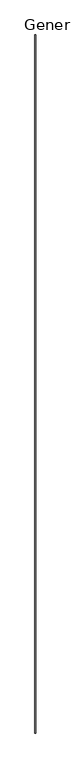
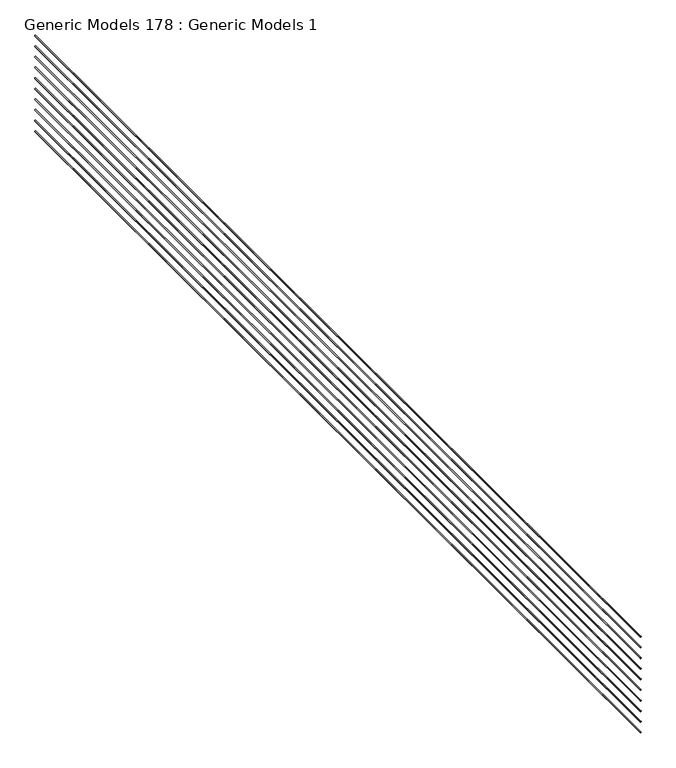
"""IFC4 building model written with IfcOpenShell, lengths in millimetres: proxy geometry, Generic Models 178 : Generic Models 1."""

from ifc_helpers import new_model, si_unit, point, frame, frame_2d, origin, place, context, project, spatial, circle_curve, trimmed, segment, composite_curve, outline, extrude, source, transform, mapped, element, save


def generic_models_178_generic_models_1_a25d1686(model_context):
    return source(origin(), model_context, "Body", "SweptSolid", [
        extrude(outline(composite_curve([segment(trimmed(circle_curve(frame_2d((124046.2609874, -10339.2972239)), 4.7625), [point((124046.2609874, -10344.0597239))], [point((124046.2609874, -10334.5347239))], False, "CARTESIAN"), True, "CONTINUOUS"), segment(trimmed(circle_curve(frame_2d((124046.2609874, -10339.2972239)), 4.7625), [point((124046.2609874, -10334.5347239))], [point((124046.2609874, -10344.0597239))], False, "CARTESIAN"), True, "CONTINUOUS")], self_intersect=False)), frame((0.0, -654.6230338, 0.0), z_axis=(0.0, 1.0, 0.0), x_axis=(0.0, 0.0, 1.0)), (0.0, 0.0, 1.0), 9475.7774227),
        extrude(outline(composite_curve([segment(trimmed(circle_curve(frame_2d((123944.6609874, -10339.2972239)), 4.7625), [point((123944.6609874, -10344.0597239))], [point((123944.6609874, -10334.5347239))], False, "CARTESIAN"), True, "CONTINUOUS"), segment(trimmed(circle_curve(frame_2d((123944.6609874, -10339.2972239)), 4.7625), [point((123944.6609874, -10334.5347239))], [point((123944.6609874, -10344.0597239))], False, "CARTESIAN"), True, "CONTINUOUS")], self_intersect=False)), frame((0.0, -654.6230338, 0.0), z_axis=(0.0, 1.0, 0.0), x_axis=(0.0, 0.0, 1.0)), (0.0, 0.0, 1.0), 9475.7774227),
        extrude(outline(composite_curve([segment(trimmed(circle_curve(frame_2d((123843.0609874, -10339.2972239)), 4.7625), [point((123843.0609874, -10344.0597239))], [point((123843.0609874, -10334.5347239))], False, "CARTESIAN"), True, "CONTINUOUS"), segment(trimmed(circle_curve(frame_2d((123843.0609874, -10339.2972239)), 4.7625), [point((123843.0609874, -10334.5347239))], [point((123843.0609874, -10344.0597239))], False, "CARTESIAN"), True, "CONTINUOUS")], self_intersect=False)), frame((0.0, -654.6230338, 0.0), z_axis=(0.0, 1.0, 0.0), x_axis=(0.0, 0.0, 1.0)), (0.0, 0.0, 1.0), 9475.7774227),
        extrude(outline(composite_curve([segment(trimmed(circle_curve(frame_2d((123741.4609874, -10339.2972239)), 4.7625), [point((123741.4609874, -10344.0597239))], [point((123741.4609874, -10334.5347239))], False, "CARTESIAN"), True, "CONTINUOUS"), segment(trimmed(circle_curve(frame_2d((123741.4609874, -10339.2972239)), 4.7625), [point((123741.4609874, -10334.5347239))], [point((123741.4609874, -10344.0597239))], False, "CARTESIAN"), True, "CONTINUOUS")], self_intersect=False)), frame((0.0, -654.6230338, 0.0), z_axis=(0.0, 1.0, 0.0), x_axis=(0.0, 0.0, 1.0)), (0.0, 0.0, 1.0), 9475.7774227),
        extrude(outline(composite_curve([segment(trimmed(circle_curve(frame_2d((123639.8609874, -10339.2972239)), 4.7625), [point((123639.8609874, -10344.0597239))], [point((123639.8609874, -10334.5347239))], False, "CARTESIAN"), True, "CONTINUOUS"), segment(trimmed(circle_curve(frame_2d((123639.8609874, -10339.2972239)), 4.7625), [point((123639.8609874, -10334.5347239))], [point((123639.8609874, -10344.0597239))], False, "CARTESIAN"), True, "CONTINUOUS")], self_intersect=False)), frame((0.0, -654.6230338, 0.0), z_axis=(0.0, 1.0, 0.0), x_axis=(0.0, 0.0, 1.0)), (0.0, 0.0, 1.0), 9475.7774227),
        extrude(outline(composite_curve([segment(trimmed(circle_curve(frame_2d((123538.2609874, -10339.2972239)), 4.7625), [point((123538.2609874, -10344.0597239))], [point((123538.2609874, -10334.5347239))], False, "CARTESIAN"), True, "CONTINUOUS"), segment(trimmed(circle_curve(frame_2d((123538.2609874, -10339.2972239)), 4.7625), [point((123538.2609874, -10334.5347239))], [point((123538.2609874, -10344.0597239))], False, "CARTESIAN"), True, "CONTINUOUS")], self_intersect=False)), frame((0.0, -654.6230338, 0.0), z_axis=(0.0, 1.0, 0.0), x_axis=(0.0, 0.0, 1.0)), (0.0, 0.0, 1.0), 9475.7774227),
        extrude(outline(composite_curve([segment(trimmed(circle_curve(frame_2d((123436.6609874, -10339.2972239)), 4.7625), [point((123436.6609874, -10344.0597239))], [point((123436.6609874, -10334.5347239))], False, "CARTESIAN"), True, "CONTINUOUS"), segment(trimmed(circle_curve(frame_2d((123436.6609874, -10339.2972239)), 4.7625), [point((123436.6609874, -10334.5347239))], [point((123436.6609874, -10344.0597239))], False, "CARTESIAN"), True, "CONTINUOUS")], self_intersect=False)), frame((0.0, -654.6230338, 0.0), z_axis=(0.0, 1.0, 0.0), x_axis=(0.0, 0.0, 1.0)), (0.0, 0.0, 1.0), 9475.7774227),
        extrude(outline(composite_curve([segment(trimmed(circle_curve(frame_2d((123335.0609874, -10339.2972239)), 4.7625), [point((123335.0609874, -10344.0597239))], [point((123335.0609874, -10334.5347239))], False, "CARTESIAN"), True, "CONTINUOUS"), segment(trimmed(circle_curve(frame_2d((123335.0609874, -10339.2972239)), 4.7625), [point((123335.0609874, -10334.5347239))], [point((123335.0609874, -10344.0597239))], False, "CARTESIAN"), True, "CONTINUOUS")], self_intersect=False)), frame((0.0, -654.6230338, 0.0), z_axis=(0.0, 1.0, 0.0), x_axis=(0.0, 0.0, 1.0)), (0.0, 0.0, 1.0), 9475.7774227),
        extrude(outline(composite_curve([segment(trimmed(circle_curve(frame_2d((123233.4609874, -10339.2972239)), 4.7625), [point((123233.4609874, -10344.0597239))], [point((123233.4609874, -10334.5347239))], False, "CARTESIAN"), True, "CONTINUOUS"), segment(trimmed(circle_curve(frame_2d((123233.4609874, -10339.2972239)), 4.7625), [point((123233.4609874, -10334.5347239))], [point((123233.4609874, -10344.0597239))], False, "CARTESIAN"), True, "CONTINUOUS")], self_intersect=False)), frame((0.0, -654.6230338, 0.0), z_axis=(0.0, 1.0, 0.0), x_axis=(0.0, 0.0, 1.0)), (0.0, 0.0, 1.0), 9475.7774227),
        extrude(outline(composite_curve([segment(trimmed(circle_curve(frame_2d((123131.8609874, -10339.2972239)), 4.7625), [point((123131.8609874, -10344.0597239))], [point((123131.8609874, -10334.5347239))], False, "CARTESIAN"), True, "CONTINUOUS"), segment(trimmed(circle_curve(frame_2d((123131.8609874, -10339.2972239)), 4.7625), [point((123131.8609874, -10334.5347239))], [point((123131.8609874, -10344.0597239))], False, "CARTESIAN"), True, "CONTINUOUS")], self_intersect=False)), frame((0.0, -654.6230338, 0.0), z_axis=(0.0, 1.0, 0.0), x_axis=(0.0, 0.0, 1.0)), (0.0, 0.0, 1.0), 9475.7774227),
    ])


if __name__ == "__main__":
    model = new_model("IFC4")
    model_context = context("Model", 3, world=origin())
    ifc_project = project(units=[si_unit("LENGTHUNIT", "METRE", prefix="MILLI")], contexts=[model_context])
    site = spatial("IfcSite", under=ifc_project)
    building = spatial("IfcBuilding", under=site)
    placement = place(None, origin())
    generic_models_178_generic_models_1_shape = generic_models_178_generic_models_1_a25d1686(model_context)
    element("IfcBuildingElementProxy", 1, Name="Generic Models 178 : Generic Models 1", ObjectType="Generic Models 178 : Generic Models 1", at=placement, inside=building, context=model_context, shape_type="MappedRepresentation", body=[
        mapped(generic_models_178_generic_models_1_shape, transform((0.0, 0.0, 0.0), x_axis=(1.0, 0.0, 0.0), y_axis=(0.0, 1.0, 0.0), z_axis=(0.0, 0.0, 1.0))),
    ])
    save(model, "model.ifc")

# Revit data of these elements
# Element 1 (IfcBuildingElementProxy, "Generic Models 178 : Generic Models 1")
#   Materials on its faces: "_1/2\" DIA. SOLID STOCK STEEL HORIZONTAL RAILINGS"
# Materials
#   "_1/2\" DIA. SOLID STOCK STEEL HORIZONTAL RAILINGS": class "Metal", colour RGB 199 199 199, transparency 0, Description = "Structural steel 50ksi", Cost = 0
